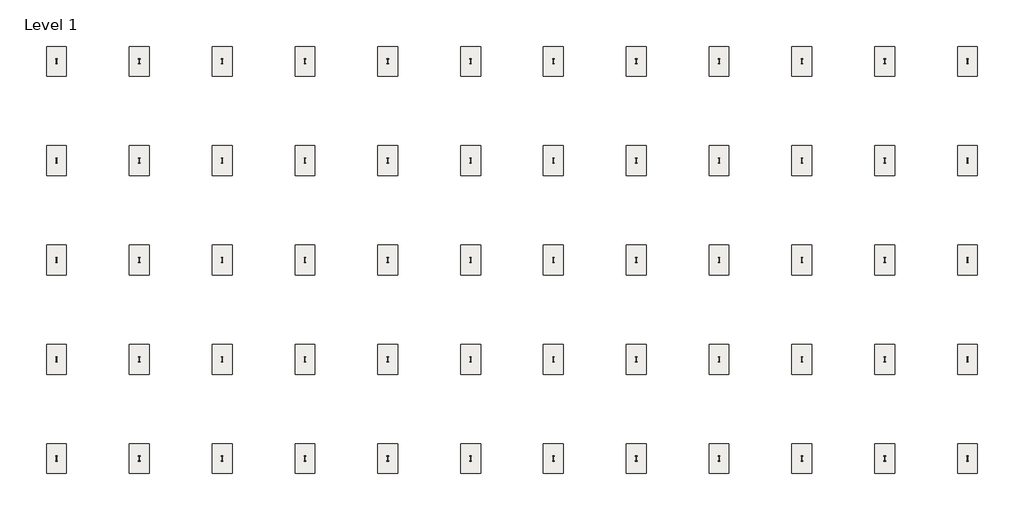
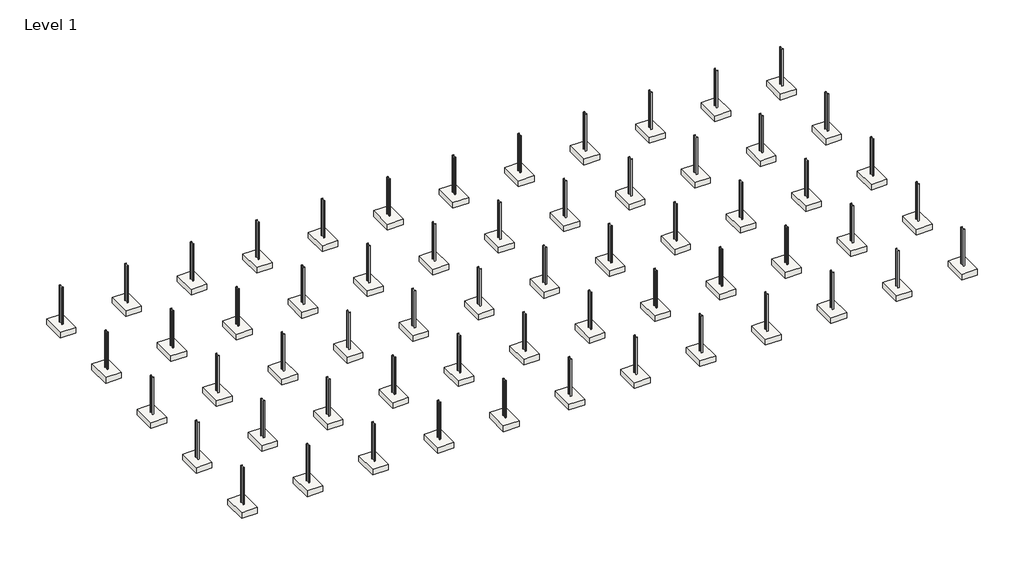
# One storey: 60 columns, 60 slabs.
"""IFC4 building model written with IfcOpenShell, lengths in millimetres."""

import ifcopenshell
import ifcopenshell.guid

model = None  # the IFC model being written
_history = None  # IfcOwnerHistory: only IFC2X3 demands one
_inside = {}  # id of a spatial element -> (the spatial element, [elements in it])
_under = {}  # id of a project, library or spatial element -> (it, [spatial elements below it])
_declared = {}  # id of a project -> (the project, [libraries it declares])
_typed = {}  # id of a type object -> (the type object, [elements of that type])
_made_of = {}  # id of a material, layer set ... -> (it, [elements and type objects made of it])


def new_model(schema):
    """Start an empty IFC model of exactly this schema.

    Asked for "IFC4X3", IfcOpenShell would pick the latest addendum, in which some entities
    have other attributes; the version numbers below select the first issue.
    IFC2X3 requires an IfcOwnerHistory on every rooted entity: one is made here for all.
    """
    global model, _history
    if schema == "IFC4X3":
        model = ifcopenshell.file(schema_version=(4, 3, 0, 0))
    else:
        model = ifcopenshell.file(schema=schema)
    _inside.clear()
    _under.clear()
    _declared.clear()
    _typed.clear()
    _made_of.clear()
    _history = None
    if model.schema == "IFC2X3":
        org = make("IfcOrganization", Name="unknown")
        user = make(
            "IfcPersonAndOrganization",
            ThePerson=make("IfcPerson", FamilyName="unknown"),
            TheOrganization=org,
        )
        app = make(
            "IfcApplication",
            ApplicationDeveloper=org,
            Version="unknown",
            ApplicationFullName="unknown",
            ApplicationIdentifier="unknown",
        )
        _history = make(
            "IfcOwnerHistory",
            OwningUser=user,
            OwningApplication=app,
            ChangeAction="ADDED",
            CreationDate=0,
        )
    return model


def make(cls, **values):
    """One entity of the class cls with the attributes given. An attribute that is None is left unset."""
    return model.create_entity(
        cls, **{name: value for name, value in values.items() if value is not None}
    )


def rooted(cls, **values):
    """An entity with a GlobalId (a new one), such as an element, a storey or a relation."""
    return make(cls, GlobalId=ifcopenshell.guid.new(), OwnerHistory=_history, **values)


def si_unit(unit_type, name, prefix=None):
    """IfcSIUnit, for example si_unit("LENGTHUNIT", "METRE", prefix="MILLI")."""
    return make("IfcSIUnit", UnitType=unit_type, Prefix=prefix, Name=name)


def assignment(units):
    """IfcUnitAssignment: the units of a project."""
    return None if units is None else make("IfcUnitAssignment", Units=units)


def point(xyz):
    """IfcCartesianPoint."""
    return None if xyz is None else make("IfcCartesianPoint", Coordinates=xyz)


def direction(xyz):
    """IfcDirection."""
    return None if xyz is None else make("IfcDirection", DirectionRatios=xyz)


def frame(location, z_axis=None, x_axis=None):
    """IfcAxis2Placement3D, a coordinate frame: its origin and axes. An axis left out is left unset."""
    return make(
        "IfcAxis2Placement3D",
        Location=point(location),
        Axis=direction(z_axis),
        RefDirection=direction(x_axis),
    )


def frame_2d(location, x_axis=None):
    """IfcAxis2Placement2D, a coordinate frame in the plane: its origin and x axis."""
    return make(
        "IfcAxis2Placement2D", Location=point(location), RefDirection=direction(x_axis)
    )


def origin():
    """The frame at (0, 0, 0) with its axes left unset."""
    return frame((0.0, 0.0, 0.0))


def origin_with_axes():
    """The frame at (0, 0, 0) with the z axis (0, 0, 1) and the x axis (1, 0, 0) written out."""
    return frame((0.0, 0.0, 0.0), z_axis=(0.0, 0.0, 1.0), x_axis=(1.0, 0.0, 0.0))


def place(relative_to, where):
    """IfcLocalPlacement: puts the frame where relative to a parent placement (None: the world)."""
    return make(
        "IfcLocalPlacement", PlacementRelTo=relative_to, RelativePlacement=where
    )


def context(
    kind, dimensions, precision=None, world=None, true_north=None, identifier=None
):
    """IfcGeometricRepresentationContext, for example the 3D "Model" context."""
    return make(
        "IfcGeometricRepresentationContext",
        ContextIdentifier=identifier,
        ContextType=kind,
        CoordinateSpaceDimension=dimensions,
        Precision=precision,
        WorldCoordinateSystem=world,
        TrueNorth=true_north,
    )


def project(units=None, contexts=None):
    """IfcProject with its units and contexts."""
    return rooted(
        "IfcProject",
        Name="project",
        RepresentationContexts=contexts,
        UnitsInContext=assignment(units),
    )


def spatial(cls, under=None, at=None, **own):
    """A site, building, storey or space (cls), placed at a placement, below another one or the project."""
    s = rooted(cls, ObjectPlacement=at, **own)
    if under is not None:
        _under.setdefault(under.id(), (under, []))[1].append(s)
    return s


def polyline(points):
    """IfcPolyline through the points."""
    return make("IfcPolyline", Points=[point(p) for p in points])


def circle_curve(where, radius):
    """IfcCircle in the frame where."""
    return make("IfcCircle", Position=where, Radius=radius)


def trimmed(basis, trim1, trim2, sense, master):
    """IfcTrimmedCurve: the piece of a basis curve between two trims."""
    return make(
        "IfcTrimmedCurve",
        BasisCurve=basis,
        Trim1=trim1,
        Trim2=trim2,
        SenseAgreement=sense,
        MasterRepresentation=master,
    )


def segment(curve, same_sense, transition):
    """IfcCompositeCurveSegment."""
    return make(
        "IfcCompositeCurveSegment",
        Transition=transition,
        SameSense=same_sense,
        ParentCurve=curve,
    )


def composite_curve(segments, self_intersect=None):
    """IfcCompositeCurve: segments joined end to end."""
    return make("IfcCompositeCurve", Segments=segments, SelfIntersect=self_intersect)


def outline(outer, holes=None, kind="AREA"):
    """IfcArbitraryClosedProfileDef: a profile drawn as a closed curve; with holes, ...WithVoids."""
    if holes is None:
        return make("IfcArbitraryClosedProfileDef", ProfileType=kind, OuterCurve=outer)
    return make(
        "IfcArbitraryProfileDefWithVoids",
        ProfileType=kind,
        OuterCurve=outer,
        InnerCurves=holes,
    )


def extrude(swept, where, along, depth):
    """IfcExtrudedAreaSolid: the profile swept, set in the frame where, extruded along a direction by depth."""
    return make(
        "IfcExtrudedAreaSolid",
        SweptArea=swept,
        Position=where,
        ExtrudedDirection=direction(along),
        Depth=depth,
    )


def shape(context_of_items, identifier, shape_type, items):
    """IfcShapeRepresentation: the items that make up one representation, for example the "Body"."""
    return make(
        "IfcShapeRepresentation",
        ContextOfItems=context_of_items,
        RepresentationIdentifier=identifier,
        RepresentationType=shape_type,
        Items=items,
    )


def source(mapping_origin, context_of_items, identifier, shape_type, items):
    """IfcRepresentationMap: a shape defined once, which mapped items show again and again."""
    return make(
        "IfcRepresentationMap",
        MappingOrigin=mapping_origin,
        MappedRepresentation=shape(context_of_items, identifier, shape_type, items),
    )


def transform(
    local_origin,
    x_axis=None,
    y_axis=None,
    z_axis=None,
    scale=None,
    scale2=None,
    scale3=None,
    uniform=True,
):
    """IfcCartesianTransformationOperator3D, or its non-uniform kind. x_axis, y_axis, z_axis: its Axis1, 2, 3."""
    if uniform:
        return make(
            "IfcCartesianTransformationOperator3D",
            Axis1=direction(x_axis),
            Axis2=direction(y_axis),
            LocalOrigin=point(local_origin),
            Scale=scale,
            Axis3=direction(z_axis),
        )
    return make(
        "IfcCartesianTransformationOperator3DnonUniform",
        Axis1=direction(x_axis),
        Axis2=direction(y_axis),
        LocalOrigin=point(local_origin),
        Scale=scale,
        Axis3=direction(z_axis),
        Scale2=scale2,
        Scale3=scale3,
    )


def mapped(mapping_source, mapping_target):
    """IfcMappedItem: shows the shape of a source again, moved by a transform."""
    return make(
        "IfcMappedItem", MappingSource=mapping_source, MappingTarget=mapping_target
    )


def made_of(thing, what):
    """Note that an element or type object is made of a material, layer set ...; save() writes the relation."""
    if what is not None:
        _made_of.setdefault(what.id(), (what, []))[1].append(thing)
    return thing


def element(
    cls,
    number,
    at=None,
    inside=None,
    cuts=None,
    type_object=None,
    material=None,
    context=None,
    identifier="Body",
    shape_type=None,
    held_by="IfcProductDefinitionShape",
    body=None,
    shapes=None,
    **own,
):
    """One element of the class cls, such as IfcWall. Its Tag is "e" and its number.

    at: its placement. inside: the storey or other place that contains it. cuts: it is an
    opening in that element (IfcRelVoidsElement). A single representation is given by context,
    identifier, shape_type and body (its items); several are given by shapes. held_by: the class
    of the entity that holds the representations. save() writes the other relations.
    """
    e = rooted(cls, Tag="e%d" % number, ObjectPlacement=at, **own)
    if body is not None:
        shapes = [shape(context, identifier, shape_type, body)]
    if shapes is not None:
        e.Representation = make(held_by, Representations=shapes)
    if inside is not None:
        _inside.setdefault(inside.id(), (inside, []))[1].append(e)
    if cuts is not None:
        rooted(
            "IfcRelVoidsElement", RelatingBuildingElement=cuts, RelatedOpeningElement=e
        )
    if type_object is not None:
        _typed.setdefault(type_object.id(), (type_object, []))[1].append(e)
    return made_of(e, material)


def aggregate(whole, parts):
    """IfcRelAggregates: a whole, such as a stair, and the parts it consists of."""
    return rooted("IfcRelAggregates", RelatingObject=whole, RelatedObjects=parts)


def save(model, path):
    """Write the relations noted so far, then the file.

    IfcRelAggregates (storeys below a building ...), IfcRelContainedInSpatialStructure (elements
    in a storey), IfcRelDefinesByType, IfcRelAssociatesMaterial and IfcRelDeclares: one each for
    every whole, place, type object, material and project.
    """
    for whole, parts in _under.values():
        aggregate(whole, parts)
    for where, things in _inside.values():
        rooted(
            "IfcRelContainedInSpatialStructure",
            RelatedElements=things,
            RelatingStructure=where,
        )
    for kind, things in _typed.values():
        rooted("IfcRelDefinesByType", RelatedObjects=things, RelatingType=kind)
    for what, things in _made_of.values():
        rooted("IfcRelAssociatesMaterial", RelatedObjects=things, RelatingMaterial=what)
    for by, libraries in _declared.values():
        rooted("IfcRelDeclares", RelatingContext=by, RelatedDefinitions=libraries)
    model.write(path)


def ub_universal_beams_column_ub305x102x25_abf45cfe(model_context):
    return source(origin(), model_context, "Body", "SweptSolid", [
        extrude(outline(composite_curve([segment(polyline([(50.8, 152.55), (50.8, 145.55), (10.5, 145.55)]), True, "CONTINUOUS"), segment(trimmed(circle_curve(frame_2d((10.5, 137.95)), 7.6), [point((10.5, 145.55))], [point((2.9, 137.95))], True, "CARTESIAN"), True, "CONTINUOUS"), segment(polyline([(2.9, 137.95), (2.9, -137.95)]), True, "CONTINUOUS"), segment(trimmed(circle_curve(frame_2d((10.5, -137.95)), 7.6), [point((2.9, -137.95))], [point((10.5, -145.55))], True, "CARTESIAN"), True, "CONTINUOUS"), segment(polyline([(10.5, -145.55), (50.8, -145.55), (50.8, -152.55), (-50.8, -152.55), (-50.8, -145.55), (-10.5, -145.55)]), True, "CONTINUOUS"), segment(trimmed(circle_curve(frame_2d((-10.5, -137.95)), 7.6), [point((-10.5, -145.55))], [point((-2.9, -137.95))], True, "CARTESIAN"), True, "CONTINUOUS"), segment(polyline([(-2.9, -137.95), (-2.9, 137.95)]), True, "CONTINUOUS"), segment(trimmed(circle_curve(frame_2d((-10.5, 137.95)), 7.6), [point((-2.9, 137.95))], [point((-10.5, 145.55))], True, "CARTESIAN"), True, "CONTINUOUS"), segment(polyline([(-10.5, 145.55), (-50.8, 145.55), (-50.8, 152.55), (50.8, 152.55)]), True, "CONTINUOUS")], self_intersect=False)), origin_with_axes(), (0.0, 0.0, 1.0), 3000.0),
    ])


def footing_rectangular_1800_x_1200_x_450mm_16ba7ea5(model_context):
    return source(origin(), model_context, "Body", "SweptSolid", [
        extrude(outline(polyline([(600.0, 900.0), (600.0, -900.0), (-600.0, -900.0), (-600.0, 900.0), (600.0, 900.0)])), frame((0.0, 0.0, -450.0), z_axis=(0.0, 0.0, 1.0), x_axis=(1.0, 0.0, 0.0)), (0.0, 0.0, 1.0), 450.0),
    ])


model = new_model("IFC4")

# Units and contexts
model_context = context("Model", 3, world=origin())
ifc_project = project(units=[si_unit("LENGTHUNIT", "METRE", prefix="MILLI")], contexts=[model_context])

# Site, building, storey
site = spatial("IfcSite", under=ifc_project)
building = spatial("IfcBuilding", under=site)
storey = spatial("IfcBuildingStorey", under=building, Name="Level 1", Elevation=0.0)

# Columns
placement = place(None, origin())
ub_universal_beams_column_ub305x102x25_shape = ub_universal_beams_column_ub305x102x25_abf45cfe(model_context)
element("IfcColumn", 1, ObjectType="UB-Universal Beams-Column : UB305x102x25", at=placement, inside=storey, context=model_context, shape_type="MappedRepresentation", body=[
    mapped(ub_universal_beams_column_ub305x102x25_shape, transform((0.0, 0.0, 0.0), x_axis=(-1.0, 0.0, 0.0), y_axis=(0.0, -1.0, 0.0), z_axis=(0.0, 0.0, 1.0))),
])
element("IfcColumn", 2, ObjectType="UB-Universal Beams-Column : UB305x102x25", at=placement, inside=storey, context=model_context, shape_type="MappedRepresentation", body=[
    mapped(ub_universal_beams_column_ub305x102x25_shape, transform((0.0, 6000.0, 0.0), x_axis=(-1.0, 0.0, 0.0), y_axis=(0.0, -1.0, 0.0), z_axis=(0.0, 0.0, 1.0))),
])
element("IfcColumn", 3, ObjectType="UB-Universal Beams-Column : UB305x102x25", at=placement, inside=storey, context=model_context, shape_type="MappedRepresentation", body=[
    mapped(ub_universal_beams_column_ub305x102x25_shape, transform((0.0, 12000.0, 0.0), x_axis=(-1.0, 0.0, 0.0), y_axis=(0.0, -1.0, 0.0), z_axis=(0.0, 0.0, 1.0))),
])
element("IfcColumn", 4, ObjectType="UB-Universal Beams-Column : UB305x102x25", at=placement, inside=storey, context=model_context, shape_type="MappedRepresentation", body=[
    mapped(ub_universal_beams_column_ub305x102x25_shape, transform((0.0, 18000.0, 0.0), x_axis=(-1.0, 0.0, 0.0), y_axis=(0.0, -1.0, 0.0), z_axis=(0.0, 0.0, 1.0))),
])
element("IfcColumn", 5, ObjectType="UB-Universal Beams-Column : UB305x102x25", at=placement, inside=storey, context=model_context, shape_type="MappedRepresentation", body=[
    mapped(ub_universal_beams_column_ub305x102x25_shape, transform((0.0, 24000.0, 0.0), x_axis=(-1.0, 0.0, 0.0), y_axis=(0.0, -1.0, 0.0), z_axis=(0.0, 0.0, 1.0))),
])
element("IfcColumn", 6, ObjectType="UB-Universal Beams-Column : UB305x102x25", at=placement, inside=storey, context=model_context, shape_type="MappedRepresentation", body=[
    mapped(ub_universal_beams_column_ub305x102x25_shape, transform((5000.0, 0.0, 0.0), x_axis=(-1.0, 0.0, 0.0), y_axis=(0.0, -1.0, 0.0), z_axis=(0.0, 0.0, 1.0))),
])
element("IfcColumn", 7, ObjectType="UB-Universal Beams-Column : UB305x102x25", at=placement, inside=storey, context=model_context, shape_type="MappedRepresentation", body=[
    mapped(ub_universal_beams_column_ub305x102x25_shape, transform((10000.0, 0.0, 0.0), x_axis=(-1.0, 0.0, 0.0), y_axis=(0.0, -1.0, 0.0), z_axis=(0.0, 0.0, 1.0))),
])
element("IfcColumn", 8, ObjectType="UB-Universal Beams-Column : UB305x102x25", at=placement, inside=storey, context=model_context, shape_type="MappedRepresentation", body=[
    mapped(ub_universal_beams_column_ub305x102x25_shape, transform((15000.0, 0.0, 0.0), x_axis=(-1.0, 0.0, 0.0), y_axis=(0.0, -1.0, 0.0), z_axis=(0.0, 0.0, 1.0))),
])
element("IfcColumn", 9, ObjectType="UB-Universal Beams-Column : UB305x102x25", at=placement, inside=storey, context=model_context, shape_type="MappedRepresentation", body=[
    mapped(ub_universal_beams_column_ub305x102x25_shape, transform((20000.0, 0.0, 0.0), x_axis=(-1.0, 0.0, 0.0), y_axis=(0.0, -1.0, 0.0), z_axis=(0.0, 0.0, 1.0))),
])
element("IfcColumn", 10, ObjectType="UB-Universal Beams-Column : UB305x102x25", at=placement, inside=storey, context=model_context, shape_type="MappedRepresentation", body=[
    mapped(ub_universal_beams_column_ub305x102x25_shape, transform((25000.0, 0.0, 0.0), x_axis=(-1.0, 0.0, 0.0), y_axis=(0.0, -1.0, 0.0), z_axis=(0.0, 0.0, 1.0))),
])
element("IfcColumn", 11, ObjectType="UB-Universal Beams-Column : UB305x102x25", at=placement, inside=storey, context=model_context, shape_type="MappedRepresentation", body=[
    mapped(ub_universal_beams_column_ub305x102x25_shape, transform((30000.0, 0.0, 0.0), x_axis=(-1.0, 0.0, 0.0), y_axis=(0.0, -1.0, 0.0), z_axis=(0.0, 0.0, 1.0))),
])
element("IfcColumn", 12, ObjectType="UB-Universal Beams-Column : UB305x102x25", at=placement, inside=storey, context=model_context, shape_type="MappedRepresentation", body=[
    mapped(ub_universal_beams_column_ub305x102x25_shape, transform((35000.0, 0.0, 0.0), x_axis=(-1.0, 0.0, 0.0), y_axis=(0.0, -1.0, 0.0), z_axis=(0.0, 0.0, 1.0))),
])
element("IfcColumn", 13, ObjectType="UB-Universal Beams-Column : UB305x102x25", at=placement, inside=storey, context=model_context, shape_type="MappedRepresentation", body=[
    mapped(ub_universal_beams_column_ub305x102x25_shape, transform((40000.0, 0.0, 0.0), x_axis=(-1.0, 0.0, 0.0), y_axis=(0.0, -1.0, 0.0), z_axis=(0.0, 0.0, 1.0))),
])
element("IfcColumn", 14, ObjectType="UB-Universal Beams-Column : UB305x102x25", at=placement, inside=storey, context=model_context, shape_type="MappedRepresentation", body=[
    mapped(ub_universal_beams_column_ub305x102x25_shape, transform((45000.0, 0.0, 0.0), x_axis=(-1.0, 0.0, 0.0), y_axis=(0.0, -1.0, 0.0), z_axis=(0.0, 0.0, 1.0))),
])
element("IfcColumn", 15, ObjectType="UB-Universal Beams-Column : UB305x102x25", at=placement, inside=storey, context=model_context, shape_type="MappedRepresentation", body=[
    mapped(ub_universal_beams_column_ub305x102x25_shape, transform((50000.0, 0.0, 0.0), x_axis=(-1.0, 0.0, 0.0), y_axis=(0.0, -1.0, 0.0), z_axis=(0.0, 0.0, 1.0))),
])
element("IfcColumn", 16, ObjectType="UB-Universal Beams-Column : UB305x102x25", at=placement, inside=storey, context=model_context, shape_type="MappedRepresentation", body=[
    mapped(ub_universal_beams_column_ub305x102x25_shape, transform((55000.0, 0.0, 0.0), x_axis=(-1.0, 0.0, 0.0), y_axis=(0.0, -1.0, 0.0), z_axis=(0.0, 0.0, 1.0))),
])
element("IfcColumn", 17, ObjectType="UB-Universal Beams-Column : UB305x102x25", at=placement, inside=storey, context=model_context, shape_type="MappedRepresentation", body=[
    mapped(ub_universal_beams_column_ub305x102x25_shape, transform((5000.0, 6000.0, 0.0), x_axis=(-1.0, 0.0, 0.0), y_axis=(0.0, -1.0, 0.0), z_axis=(0.0, 0.0, 1.0))),
])
element("IfcColumn", 18, ObjectType="UB-Universal Beams-Column : UB305x102x25", at=placement, inside=storey, context=model_context, shape_type="MappedRepresentation", body=[
    mapped(ub_universal_beams_column_ub305x102x25_shape, transform((5000.0, 12000.0, 0.0), x_axis=(-1.0, 0.0, 0.0), y_axis=(0.0, -1.0, 0.0), z_axis=(0.0, 0.0, 1.0))),
])
element("IfcColumn", 19, ObjectType="UB-Universal Beams-Column : UB305x102x25", at=placement, inside=storey, context=model_context, shape_type="MappedRepresentation", body=[
    mapped(ub_universal_beams_column_ub305x102x25_shape, transform((5000.0, 18000.0, 0.0), x_axis=(-1.0, 0.0, 0.0), y_axis=(0.0, -1.0, 0.0), z_axis=(0.0, 0.0, 1.0))),
])
element("IfcColumn", 20, ObjectType="UB-Universal Beams-Column : UB305x102x25", at=placement, inside=storey, context=model_context, shape_type="MappedRepresentation", body=[
    mapped(ub_universal_beams_column_ub305x102x25_shape, transform((5000.0, 24000.0, 0.0), x_axis=(-1.0, 0.0, 0.0), y_axis=(0.0, -1.0, 0.0), z_axis=(0.0, 0.0, 1.0))),
])
element("IfcColumn", 21, ObjectType="UB-Universal Beams-Column : UB305x102x25", at=placement, inside=storey, context=model_context, shape_type="MappedRepresentation", body=[
    mapped(ub_universal_beams_column_ub305x102x25_shape, transform((10000.0, 6000.0, 0.0), x_axis=(-1.0, 0.0, 0.0), y_axis=(0.0, -1.0, 0.0), z_axis=(0.0, 0.0, 1.0))),
])
element("IfcColumn", 22, ObjectType="UB-Universal Beams-Column : UB305x102x25", at=placement, inside=storey, context=model_context, shape_type="MappedRepresentation", body=[
    mapped(ub_universal_beams_column_ub305x102x25_shape, transform((10000.0, 12000.0, 0.0), x_axis=(-1.0, 0.0, 0.0), y_axis=(0.0, -1.0, 0.0), z_axis=(0.0, 0.0, 1.0))),
])
element("IfcColumn", 23, ObjectType="UB-Universal Beams-Column : UB305x102x25", at=placement, inside=storey, context=model_context, shape_type="MappedRepresentation", body=[
    mapped(ub_universal_beams_column_ub305x102x25_shape, transform((10000.0, 18000.0, 0.0), x_axis=(-1.0, 0.0, 0.0), y_axis=(0.0, -1.0, 0.0), z_axis=(0.0, 0.0, 1.0))),
])
element("IfcColumn", 24, ObjectType="UB-Universal Beams-Column : UB305x102x25", at=placement, inside=storey, context=model_context, shape_type="MappedRepresentation", body=[
    mapped(ub_universal_beams_column_ub305x102x25_shape, transform((10000.0, 24000.0, 0.0), x_axis=(-1.0, 0.0, 0.0), y_axis=(0.0, -1.0, 0.0), z_axis=(0.0, 0.0, 1.0))),
])
element("IfcColumn", 25, ObjectType="UB-Universal Beams-Column : UB305x102x25", at=placement, inside=storey, context=model_context, shape_type="MappedRepresentation", body=[
    mapped(ub_universal_beams_column_ub305x102x25_shape, transform((15000.0, 6000.0, 0.0), x_axis=(-1.0, 0.0, 0.0), y_axis=(0.0, -1.0, 0.0), z_axis=(0.0, 0.0, 1.0))),
])
element("IfcColumn", 26, ObjectType="UB-Universal Beams-Column : UB305x102x25", at=placement, inside=storey, context=model_context, shape_type="MappedRepresentation", body=[
    mapped(ub_universal_beams_column_ub305x102x25_shape, transform((15000.0, 12000.0, 0.0), x_axis=(-1.0, 0.0, 0.0), y_axis=(0.0, -1.0, 0.0), z_axis=(0.0, 0.0, 1.0))),
])
element("IfcColumn", 27, ObjectType="UB-Universal Beams-Column : UB305x102x25", at=placement, inside=storey, context=model_context, shape_type="MappedRepresentation", body=[
    mapped(ub_universal_beams_column_ub305x102x25_shape, transform((15000.0, 18000.0, 0.0), x_axis=(-1.0, 0.0, 0.0), y_axis=(0.0, -1.0, 0.0), z_axis=(0.0, 0.0, 1.0))),
])
element("IfcColumn", 28, ObjectType="UB-Universal Beams-Column : UB305x102x25", at=placement, inside=storey, context=model_context, shape_type="MappedRepresentation", body=[
    mapped(ub_universal_beams_column_ub305x102x25_shape, transform((15000.0, 24000.0, 0.0), x_axis=(-1.0, 0.0, 0.0), y_axis=(0.0, -1.0, 0.0), z_axis=(0.0, 0.0, 1.0))),
])
element("IfcColumn", 29, ObjectType="UB-Universal Beams-Column : UB305x102x25", at=placement, inside=storey, context=model_context, shape_type="MappedRepresentation", body=[
    mapped(ub_universal_beams_column_ub305x102x25_shape, transform((20000.0, 6000.0, 0.0), x_axis=(-1.0, 0.0, 0.0), y_axis=(0.0, -1.0, 0.0), z_axis=(0.0, 0.0, 1.0))),
])
element("IfcColumn", 30, ObjectType="UB-Universal Beams-Column : UB305x102x25", at=placement, inside=storey, context=model_context, shape_type="MappedRepresentation", body=[
    mapped(ub_universal_beams_column_ub305x102x25_shape, transform((20000.0, 12000.0, 0.0), x_axis=(-1.0, 0.0, 0.0), y_axis=(0.0, -1.0, 0.0), z_axis=(0.0, 0.0, 1.0))),
])
element("IfcColumn", 31, ObjectType="UB-Universal Beams-Column : UB305x102x25", at=placement, inside=storey, context=model_context, shape_type="MappedRepresentation", body=[
    mapped(ub_universal_beams_column_ub305x102x25_shape, transform((20000.0, 18000.0, 0.0), x_axis=(-1.0, 0.0, 0.0), y_axis=(0.0, -1.0, 0.0), z_axis=(0.0, 0.0, 1.0))),
])
element("IfcColumn", 32, ObjectType="UB-Universal Beams-Column : UB305x102x25", at=placement, inside=storey, context=model_context, shape_type="MappedRepresentation", body=[
    mapped(ub_universal_beams_column_ub305x102x25_shape, transform((20000.0, 24000.0, 0.0), x_axis=(-1.0, 0.0, 0.0), y_axis=(0.0, -1.0, 0.0), z_axis=(0.0, 0.0, 1.0))),
])
element("IfcColumn", 33, ObjectType="UB-Universal Beams-Column : UB305x102x25", at=placement, inside=storey, context=model_context, shape_type="MappedRepresentation", body=[
    mapped(ub_universal_beams_column_ub305x102x25_shape, transform((25000.0, 6000.0, 0.0), x_axis=(-1.0, 0.0, 0.0), y_axis=(0.0, -1.0, 0.0), z_axis=(0.0, 0.0, 1.0))),
])
element("IfcColumn", 34, ObjectType="UB-Universal Beams-Column : UB305x102x25", at=placement, inside=storey, context=model_context, shape_type="MappedRepresentation", body=[
    mapped(ub_universal_beams_column_ub305x102x25_shape, transform((25000.0, 12000.0, 0.0), x_axis=(-1.0, 0.0, 0.0), y_axis=(0.0, -1.0, 0.0), z_axis=(0.0, 0.0, 1.0))),
])
element("IfcColumn", 35, ObjectType="UB-Universal Beams-Column : UB305x102x25", at=placement, inside=storey, context=model_context, shape_type="MappedRepresentation", body=[
    mapped(ub_universal_beams_column_ub305x102x25_shape, transform((25000.0, 18000.0, 0.0), x_axis=(-1.0, 0.0, 0.0), y_axis=(0.0, -1.0, 0.0), z_axis=(0.0, 0.0, 1.0))),
])
element("IfcColumn", 36, ObjectType="UB-Universal Beams-Column : UB305x102x25", at=placement, inside=storey, context=model_context, shape_type="MappedRepresentation", body=[
    mapped(ub_universal_beams_column_ub305x102x25_shape, transform((25000.0, 24000.0, 0.0), x_axis=(-1.0, 0.0, 0.0), y_axis=(0.0, -1.0, 0.0), z_axis=(0.0, 0.0, 1.0))),
])
element("IfcColumn", 37, ObjectType="UB-Universal Beams-Column : UB305x102x25", at=placement, inside=storey, context=model_context, shape_type="MappedRepresentation", body=[
    mapped(ub_universal_beams_column_ub305x102x25_shape, transform((30000.0, 6000.0, 0.0), x_axis=(-1.0, 0.0, 0.0), y_axis=(0.0, -1.0, 0.0), z_axis=(0.0, 0.0, 1.0))),
])
element("IfcColumn", 38, ObjectType="UB-Universal Beams-Column : UB305x102x25", at=placement, inside=storey, context=model_context, shape_type="MappedRepresentation", body=[
    mapped(ub_universal_beams_column_ub305x102x25_shape, transform((30000.0, 12000.0, 0.0), x_axis=(-1.0, 0.0, 0.0), y_axis=(0.0, -1.0, 0.0), z_axis=(0.0, 0.0, 1.0))),
])
element("IfcColumn", 39, ObjectType="UB-Universal Beams-Column : UB305x102x25", at=placement, inside=storey, context=model_context, shape_type="MappedRepresentation", body=[
    mapped(ub_universal_beams_column_ub305x102x25_shape, transform((30000.0, 18000.0, 0.0), x_axis=(-1.0, 0.0, 0.0), y_axis=(0.0, -1.0, 0.0), z_axis=(0.0, 0.0, 1.0))),
])
element("IfcColumn", 40, ObjectType="UB-Universal Beams-Column : UB305x102x25", at=placement, inside=storey, context=model_context, shape_type="MappedRepresentation", body=[
    mapped(ub_universal_beams_column_ub305x102x25_shape, transform((30000.0, 24000.0, 0.0), x_axis=(-1.0, 0.0, 0.0), y_axis=(0.0, -1.0, 0.0), z_axis=(0.0, 0.0, 1.0))),
])
element("IfcColumn", 41, ObjectType="UB-Universal Beams-Column : UB305x102x25", at=placement, inside=storey, context=model_context, shape_type="MappedRepresentation", body=[
    mapped(ub_universal_beams_column_ub305x102x25_shape, transform((35000.0, 6000.0, 0.0), x_axis=(-1.0, 0.0, 0.0), y_axis=(0.0, -1.0, 0.0), z_axis=(0.0, 0.0, 1.0))),
])
element("IfcColumn", 42, ObjectType="UB-Universal Beams-Column : UB305x102x25", at=placement, inside=storey, context=model_context, shape_type="MappedRepresentation", body=[
    mapped(ub_universal_beams_column_ub305x102x25_shape, transform((35000.0, 12000.0, 0.0), x_axis=(-1.0, 0.0, 0.0), y_axis=(0.0, -1.0, 0.0), z_axis=(0.0, 0.0, 1.0))),
])
element("IfcColumn", 43, ObjectType="UB-Universal Beams-Column : UB305x102x25", at=placement, inside=storey, context=model_context, shape_type="MappedRepresentation", body=[
    mapped(ub_universal_beams_column_ub305x102x25_shape, transform((35000.0, 18000.0, 0.0), x_axis=(-1.0, 0.0, 0.0), y_axis=(0.0, -1.0, 0.0), z_axis=(0.0, 0.0, 1.0))),
])
element("IfcColumn", 44, ObjectType="UB-Universal Beams-Column : UB305x102x25", at=placement, inside=storey, context=model_context, shape_type="MappedRepresentation", body=[
    mapped(ub_universal_beams_column_ub305x102x25_shape, transform((35000.0, 24000.0, 0.0), x_axis=(-1.0, 0.0, 0.0), y_axis=(0.0, -1.0, 0.0), z_axis=(0.0, 0.0, 1.0))),
])
element("IfcColumn", 45, ObjectType="UB-Universal Beams-Column : UB305x102x25", at=placement, inside=storey, context=model_context, shape_type="MappedRepresentation", body=[
    mapped(ub_universal_beams_column_ub305x102x25_shape, transform((40000.0, 6000.0, 0.0), x_axis=(-1.0, 0.0, 0.0), y_axis=(0.0, -1.0, 0.0), z_axis=(0.0, 0.0, 1.0))),
])
element("IfcColumn", 46, ObjectType="UB-Universal Beams-Column : UB305x102x25", at=placement, inside=storey, context=model_context, shape_type="MappedRepresentation", body=[
    mapped(ub_universal_beams_column_ub305x102x25_shape, transform((40000.0, 12000.0, 0.0), x_axis=(-1.0, 0.0, 0.0), y_axis=(0.0, -1.0, 0.0), z_axis=(0.0, 0.0, 1.0))),
])
element("IfcColumn", 47, ObjectType="UB-Universal Beams-Column : UB305x102x25", at=placement, inside=storey, context=model_context, shape_type="MappedRepresentation", body=[
    mapped(ub_universal_beams_column_ub305x102x25_shape, transform((40000.0, 18000.0, 0.0), x_axis=(-1.0, 0.0, 0.0), y_axis=(0.0, -1.0, 0.0), z_axis=(0.0, 0.0, 1.0))),
])
element("IfcColumn", 48, ObjectType="UB-Universal Beams-Column : UB305x102x25", at=placement, inside=storey, context=model_context, shape_type="MappedRepresentation", body=[
    mapped(ub_universal_beams_column_ub305x102x25_shape, transform((40000.0, 24000.0, 0.0), x_axis=(-1.0, 0.0, 0.0), y_axis=(0.0, -1.0, 0.0), z_axis=(0.0, 0.0, 1.0))),
])
element("IfcColumn", 49, ObjectType="UB-Universal Beams-Column : UB305x102x25", at=placement, inside=storey, context=model_context, shape_type="MappedRepresentation", body=[
    mapped(ub_universal_beams_column_ub305x102x25_shape, transform((45000.0, 6000.0, 0.0), x_axis=(-1.0, 0.0, 0.0), y_axis=(0.0, -1.0, 0.0), z_axis=(0.0, 0.0, 1.0))),
])
element("IfcColumn", 50, ObjectType="UB-Universal Beams-Column : UB305x102x25", at=placement, inside=storey, context=model_context, shape_type="MappedRepresentation", body=[
    mapped(ub_universal_beams_column_ub305x102x25_shape, transform((45000.0, 12000.0, 0.0), x_axis=(-1.0, 0.0, 0.0), y_axis=(0.0, -1.0, 0.0), z_axis=(0.0, 0.0, 1.0))),
])
element("IfcColumn", 51, ObjectType="UB-Universal Beams-Column : UB305x102x25", at=placement, inside=storey, context=model_context, shape_type="MappedRepresentation", body=[
    mapped(ub_universal_beams_column_ub305x102x25_shape, transform((45000.0, 18000.0, 0.0), x_axis=(-1.0, 0.0, 0.0), y_axis=(0.0, -1.0, 0.0), z_axis=(0.0, 0.0, 1.0))),
])
element("IfcColumn", 52, ObjectType="UB-Universal Beams-Column : UB305x102x25", at=placement, inside=storey, context=model_context, shape_type="MappedRepresentation", body=[
    mapped(ub_universal_beams_column_ub305x102x25_shape, transform((45000.0, 24000.0, 0.0), x_axis=(-1.0, 0.0, 0.0), y_axis=(0.0, -1.0, 0.0), z_axis=(0.0, 0.0, 1.0))),
])
element("IfcColumn", 53, ObjectType="UB-Universal Beams-Column : UB305x102x25", at=placement, inside=storey, context=model_context, shape_type="MappedRepresentation", body=[
    mapped(ub_universal_beams_column_ub305x102x25_shape, transform((50000.0, 6000.0, 0.0), x_axis=(-1.0, 0.0, 0.0), y_axis=(0.0, -1.0, 0.0), z_axis=(0.0, 0.0, 1.0))),
])
element("IfcColumn", 54, ObjectType="UB-Universal Beams-Column : UB305x102x25", at=placement, inside=storey, context=model_context, shape_type="MappedRepresentation", body=[
    mapped(ub_universal_beams_column_ub305x102x25_shape, transform((50000.0, 12000.0, 0.0), x_axis=(-1.0, 0.0, 0.0), y_axis=(0.0, -1.0, 0.0), z_axis=(0.0, 0.0, 1.0))),
])
element("IfcColumn", 55, ObjectType="UB-Universal Beams-Column : UB305x102x25", at=placement, inside=storey, context=model_context, shape_type="MappedRepresentation", body=[
    mapped(ub_universal_beams_column_ub305x102x25_shape, transform((50000.0, 18000.0, 0.0), x_axis=(-1.0, 0.0, 0.0), y_axis=(0.0, -1.0, 0.0), z_axis=(0.0, 0.0, 1.0))),
])
element("IfcColumn", 56, ObjectType="UB-Universal Beams-Column : UB305x102x25", at=placement, inside=storey, context=model_context, shape_type="MappedRepresentation", body=[
    mapped(ub_universal_beams_column_ub305x102x25_shape, transform((50000.0, 24000.0, 0.0), x_axis=(-1.0, 0.0, 0.0), y_axis=(0.0, -1.0, 0.0), z_axis=(0.0, 0.0, 1.0))),
])
element("IfcColumn", 57, ObjectType="UB-Universal Beams-Column : UB305x102x25", at=placement, inside=storey, context=model_context, shape_type="MappedRepresentation", body=[
    mapped(ub_universal_beams_column_ub305x102x25_shape, transform((55000.0, 6000.0, 0.0), x_axis=(-1.0, 0.0, 0.0), y_axis=(0.0, -1.0, 0.0), z_axis=(0.0, 0.0, 1.0))),
])
element("IfcColumn", 58, ObjectType="UB-Universal Beams-Column : UB305x102x25", at=placement, inside=storey, context=model_context, shape_type="MappedRepresentation", body=[
    mapped(ub_universal_beams_column_ub305x102x25_shape, transform((55000.0, 12000.0, 0.0), x_axis=(-1.0, 0.0, 0.0), y_axis=(0.0, -1.0, 0.0), z_axis=(0.0, 0.0, 1.0))),
])
element("IfcColumn", 59, ObjectType="UB-Universal Beams-Column : UB305x102x25", at=placement, inside=storey, context=model_context, shape_type="MappedRepresentation", body=[
    mapped(ub_universal_beams_column_ub305x102x25_shape, transform((55000.0, 18000.0, 0.0), x_axis=(-1.0, 0.0, 0.0), y_axis=(0.0, -1.0, 0.0), z_axis=(0.0, 0.0, 1.0))),
])
element("IfcColumn", 60, ObjectType="UB-Universal Beams-Column : UB305x102x25", at=placement, inside=storey, context=model_context, shape_type="MappedRepresentation", body=[
    mapped(ub_universal_beams_column_ub305x102x25_shape, transform((55000.0, 24000.0, 0.0), x_axis=(-1.0, 0.0, 0.0), y_axis=(0.0, -1.0, 0.0), z_axis=(0.0, 0.0, 1.0))),
])

# Slabs
footing_rectangular_1800_x_1200_x_450mm_shape = footing_rectangular_1800_x_1200_x_450mm_16ba7ea5(model_context)
element("IfcSlab", 61, ObjectType="Footing-Rectangular : 1800 x 1200 x 450mm", at=placement, inside=storey, context=model_context, shape_type="MappedRepresentation", body=[
    mapped(footing_rectangular_1800_x_1200_x_450mm_shape, transform((0.0, 24000.0, 0.0), x_axis=(1.0, 0.0, 0.0), y_axis=(0.0, 1.0, 0.0), z_axis=(0.0, 0.0, 1.0))),
])
element("IfcSlab", 62, ObjectType="Footing-Rectangular : 1800 x 1200 x 450mm", at=placement, inside=storey, context=model_context, shape_type="MappedRepresentation", body=[
    mapped(footing_rectangular_1800_x_1200_x_450mm_shape, transform((5000.0, 24000.0, 0.0), x_axis=(1.0, 0.0, 0.0), y_axis=(0.0, 1.0, 0.0), z_axis=(0.0, 0.0, 1.0))),
])
element("IfcSlab", 63, ObjectType="Footing-Rectangular : 1800 x 1200 x 450mm", at=placement, inside=storey, context=model_context, shape_type="MappedRepresentation", body=[
    mapped(footing_rectangular_1800_x_1200_x_450mm_shape, transform((10000.0, 6000.0, 0.0), x_axis=(-1.0, 0.0, 0.0), y_axis=(0.0, -1.0, 0.0), z_axis=(0.0, 0.0, 1.0))),
])
element("IfcSlab", 64, ObjectType="Footing-Rectangular : 1800 x 1200 x 450mm", at=placement, inside=storey, context=model_context, shape_type="MappedRepresentation", body=[
    mapped(footing_rectangular_1800_x_1200_x_450mm_shape, transform((10000.0, 12000.0, 0.0), x_axis=(-1.0, 0.0, 0.0), y_axis=(0.0, -1.0, 0.0), z_axis=(0.0, 0.0, 1.0))),
])
element("IfcSlab", 65, ObjectType="Footing-Rectangular : 1800 x 1200 x 450mm", at=placement, inside=storey, context=model_context, shape_type="MappedRepresentation", body=[
    mapped(footing_rectangular_1800_x_1200_x_450mm_shape, transform((10000.0, 18000.0, 0.0), x_axis=(-1.0, 0.0, 0.0), y_axis=(0.0, -1.0, 0.0), z_axis=(0.0, 0.0, 1.0))),
])
element("IfcSlab", 66, ObjectType="Footing-Rectangular : 1800 x 1200 x 450mm", at=placement, inside=storey, context=model_context, shape_type="MappedRepresentation", body=[
    mapped(footing_rectangular_1800_x_1200_x_450mm_shape, transform((10000.0, 24000.0, 0.0), x_axis=(-1.0, 0.0, 0.0), y_axis=(0.0, -1.0, 0.0), z_axis=(0.0, 0.0, 1.0))),
])
element("IfcSlab", 67, ObjectType="Footing-Rectangular : 1800 x 1200 x 450mm", at=placement, inside=storey, context=model_context, shape_type="MappedRepresentation", body=[
    mapped(footing_rectangular_1800_x_1200_x_450mm_shape, transform((15000.0, 6000.0, 0.0), x_axis=(-1.0, 0.0, 0.0), y_axis=(0.0, -1.0, 0.0), z_axis=(0.0, 0.0, 1.0))),
])
element("IfcSlab", 68, ObjectType="Footing-Rectangular : 1800 x 1200 x 450mm", at=placement, inside=storey, context=model_context, shape_type="MappedRepresentation", body=[
    mapped(footing_rectangular_1800_x_1200_x_450mm_shape, transform((15000.0, 12000.0, 0.0), x_axis=(-1.0, 0.0, 0.0), y_axis=(0.0, -1.0, 0.0), z_axis=(0.0, 0.0, 1.0))),
])
element("IfcSlab", 69, ObjectType="Footing-Rectangular : 1800 x 1200 x 450mm", at=placement, inside=storey, context=model_context, shape_type="MappedRepresentation", body=[
    mapped(footing_rectangular_1800_x_1200_x_450mm_shape, transform((15000.0, 18000.0, 0.0), x_axis=(-1.0, 0.0, 0.0), y_axis=(0.0, -1.0, 0.0), z_axis=(0.0, 0.0, 1.0))),
])
element("IfcSlab", 70, ObjectType="Footing-Rectangular : 1800 x 1200 x 450mm", at=placement, inside=storey, context=model_context, shape_type="MappedRepresentation", body=[
    mapped(footing_rectangular_1800_x_1200_x_450mm_shape, transform((15000.0, 24000.0, 0.0), x_axis=(-1.0, 0.0, 0.0), y_axis=(0.0, -1.0, 0.0), z_axis=(0.0, 0.0, 1.0))),
])
element("IfcSlab", 71, ObjectType="Footing-Rectangular : 1800 x 1200 x 450mm", at=placement, inside=storey, context=model_context, shape_type="MappedRepresentation", body=[
    mapped(footing_rectangular_1800_x_1200_x_450mm_shape, transform((20000.0, 6000.0, 0.0), x_axis=(-1.0, 0.0, 0.0), y_axis=(0.0, -1.0, 0.0), z_axis=(0.0, 0.0, 1.0))),
])
element("IfcSlab", 72, ObjectType="Footing-Rectangular : 1800 x 1200 x 450mm", at=placement, inside=storey, context=model_context, shape_type="MappedRepresentation", body=[
    mapped(footing_rectangular_1800_x_1200_x_450mm_shape, transform((20000.0, 12000.0, 0.0), x_axis=(-1.0, 0.0, 0.0), y_axis=(0.0, -1.0, 0.0), z_axis=(0.0, 0.0, 1.0))),
])
element("IfcSlab", 73, ObjectType="Footing-Rectangular : 1800 x 1200 x 450mm", at=placement, inside=storey, context=model_context, shape_type="MappedRepresentation", body=[
    mapped(footing_rectangular_1800_x_1200_x_450mm_shape, transform((20000.0, 18000.0, 0.0), x_axis=(-1.0, 0.0, 0.0), y_axis=(0.0, -1.0, 0.0), z_axis=(0.0, 0.0, 1.0))),
])
element("IfcSlab", 74, ObjectType="Footing-Rectangular : 1800 x 1200 x 450mm", at=placement, inside=storey, context=model_context, shape_type="MappedRepresentation", body=[
    mapped(footing_rectangular_1800_x_1200_x_450mm_shape, transform((20000.0, 24000.0, 0.0), x_axis=(-1.0, 0.0, 0.0), y_axis=(0.0, -1.0, 0.0), z_axis=(0.0, 0.0, 1.0))),
])
element("IfcSlab", 75, ObjectType="Footing-Rectangular : 1800 x 1200 x 450mm", at=placement, inside=storey, context=model_context, shape_type="MappedRepresentation", body=[
    mapped(footing_rectangular_1800_x_1200_x_450mm_shape, transform((25000.0, 6000.0, 0.0), x_axis=(-1.0, 0.0, 0.0), y_axis=(0.0, -1.0, 0.0), z_axis=(0.0, 0.0, 1.0))),
])
element("IfcSlab", 76, ObjectType="Footing-Rectangular : 1800 x 1200 x 450mm", at=placement, inside=storey, context=model_context, shape_type="MappedRepresentation", body=[
    mapped(footing_rectangular_1800_x_1200_x_450mm_shape, transform((25000.0, 12000.0, 0.0), x_axis=(-1.0, 0.0, 0.0), y_axis=(0.0, -1.0, 0.0), z_axis=(0.0, 0.0, 1.0))),
])
element("IfcSlab", 77, ObjectType="Footing-Rectangular : 1800 x 1200 x 450mm", at=placement, inside=storey, context=model_context, shape_type="MappedRepresentation", body=[
    mapped(footing_rectangular_1800_x_1200_x_450mm_shape, transform((25000.0, 18000.0, 0.0), x_axis=(-1.0, 0.0, 0.0), y_axis=(0.0, -1.0, 0.0), z_axis=(0.0, 0.0, 1.0))),
])
element("IfcSlab", 78, ObjectType="Footing-Rectangular : 1800 x 1200 x 450mm", at=placement, inside=storey, context=model_context, shape_type="MappedRepresentation", body=[
    mapped(footing_rectangular_1800_x_1200_x_450mm_shape, transform((25000.0, 24000.0, 0.0), x_axis=(-1.0, 0.0, 0.0), y_axis=(0.0, -1.0, 0.0), z_axis=(0.0, 0.0, 1.0))),
])
element("IfcSlab", 79, ObjectType="Footing-Rectangular : 1800 x 1200 x 450mm", at=placement, inside=storey, context=model_context, shape_type="MappedRepresentation", body=[
    mapped(footing_rectangular_1800_x_1200_x_450mm_shape, transform((30000.0, 6000.0, 0.0), x_axis=(-1.0, 0.0, 0.0), y_axis=(0.0, -1.0, 0.0), z_axis=(0.0, 0.0, 1.0))),
])
element("IfcSlab", 80, ObjectType="Footing-Rectangular : 1800 x 1200 x 450mm", at=placement, inside=storey, context=model_context, shape_type="MappedRepresentation", body=[
    mapped(footing_rectangular_1800_x_1200_x_450mm_shape, transform((30000.0, 12000.0, 0.0), x_axis=(-1.0, 0.0, 0.0), y_axis=(0.0, -1.0, 0.0), z_axis=(0.0, 0.0, 1.0))),
])
element("IfcSlab", 81, ObjectType="Footing-Rectangular : 1800 x 1200 x 450mm", at=placement, inside=storey, context=model_context, shape_type="MappedRepresentation", body=[
    mapped(footing_rectangular_1800_x_1200_x_450mm_shape, transform((30000.0, 18000.0, 0.0), x_axis=(-1.0, 0.0, 0.0), y_axis=(0.0, -1.0, 0.0), z_axis=(0.0, 0.0, 1.0))),
])
element("IfcSlab", 82, ObjectType="Footing-Rectangular : 1800 x 1200 x 450mm", at=placement, inside=storey, context=model_context, shape_type="MappedRepresentation", body=[
    mapped(footing_rectangular_1800_x_1200_x_450mm_shape, transform((30000.0, 24000.0, 0.0), x_axis=(-1.0, 0.0, 0.0), y_axis=(0.0, -1.0, 0.0), z_axis=(0.0, 0.0, 1.0))),
])
element("IfcSlab", 83, ObjectType="Footing-Rectangular : 1800 x 1200 x 450mm", at=placement, inside=storey, context=model_context, shape_type="MappedRepresentation", body=[
    mapped(footing_rectangular_1800_x_1200_x_450mm_shape, transform((35000.0, 6000.0, 0.0), x_axis=(-1.0, 0.0, 0.0), y_axis=(0.0, -1.0, 0.0), z_axis=(0.0, 0.0, 1.0))),
])
element("IfcSlab", 84, ObjectType="Footing-Rectangular : 1800 x 1200 x 450mm", at=placement, inside=storey, context=model_context, shape_type="MappedRepresentation", body=[
    mapped(footing_rectangular_1800_x_1200_x_450mm_shape, transform((35000.0, 12000.0, 0.0), x_axis=(-1.0, 0.0, 0.0), y_axis=(0.0, -1.0, 0.0), z_axis=(0.0, 0.0, 1.0))),
])
element("IfcSlab", 85, ObjectType="Footing-Rectangular : 1800 x 1200 x 450mm", at=placement, inside=storey, context=model_context, shape_type="MappedRepresentation", body=[
    mapped(footing_rectangular_1800_x_1200_x_450mm_shape, transform((35000.0, 18000.0, 0.0), x_axis=(-1.0, 0.0, 0.0), y_axis=(0.0, -1.0, 0.0), z_axis=(0.0, 0.0, 1.0))),
])
element("IfcSlab", 86, ObjectType="Footing-Rectangular : 1800 x 1200 x 450mm", at=placement, inside=storey, context=model_context, shape_type="MappedRepresentation", body=[
    mapped(footing_rectangular_1800_x_1200_x_450mm_shape, transform((35000.0, 24000.0, 0.0), x_axis=(-1.0, 0.0, 0.0), y_axis=(0.0, -1.0, 0.0), z_axis=(0.0, 0.0, 1.0))),
])
element("IfcSlab", 87, ObjectType="Footing-Rectangular : 1800 x 1200 x 450mm", at=placement, inside=storey, context=model_context, shape_type="MappedRepresentation", body=[
    mapped(footing_rectangular_1800_x_1200_x_450mm_shape, transform((40000.0, 6000.0, 0.0), x_axis=(-1.0, 0.0, 0.0), y_axis=(0.0, -1.0, 0.0), z_axis=(0.0, 0.0, 1.0))),
])
element("IfcSlab", 88, ObjectType="Footing-Rectangular : 1800 x 1200 x 450mm", at=placement, inside=storey, context=model_context, shape_type="MappedRepresentation", body=[
    mapped(footing_rectangular_1800_x_1200_x_450mm_shape, transform((40000.0, 12000.0, 0.0), x_axis=(-1.0, 0.0, 0.0), y_axis=(0.0, -1.0, 0.0), z_axis=(0.0, 0.0, 1.0))),
])
element("IfcSlab", 89, ObjectType="Footing-Rectangular : 1800 x 1200 x 450mm", at=placement, inside=storey, context=model_context, shape_type="MappedRepresentation", body=[
    mapped(footing_rectangular_1800_x_1200_x_450mm_shape, transform((40000.0, 18000.0, 0.0), x_axis=(-1.0, 0.0, 0.0), y_axis=(0.0, -1.0, 0.0), z_axis=(0.0, 0.0, 1.0))),
])
element("IfcSlab", 90, ObjectType="Footing-Rectangular : 1800 x 1200 x 450mm", at=placement, inside=storey, context=model_context, shape_type="MappedRepresentation", body=[
    mapped(footing_rectangular_1800_x_1200_x_450mm_shape, transform((40000.0, 24000.0, 0.0), x_axis=(-1.0, 0.0, 0.0), y_axis=(0.0, -1.0, 0.0), z_axis=(0.0, 0.0, 1.0))),
])
element("IfcSlab", 91, ObjectType="Footing-Rectangular : 1800 x 1200 x 450mm", at=placement, inside=storey, context=model_context, shape_type="MappedRepresentation", body=[
    mapped(footing_rectangular_1800_x_1200_x_450mm_shape, transform((45000.0, 6000.0, 0.0), x_axis=(-1.0, 0.0, 0.0), y_axis=(0.0, -1.0, 0.0), z_axis=(0.0, 0.0, 1.0))),
])
element("IfcSlab", 92, ObjectType="Footing-Rectangular : 1800 x 1200 x 450mm", at=placement, inside=storey, context=model_context, shape_type="MappedRepresentation", body=[
    mapped(footing_rectangular_1800_x_1200_x_450mm_shape, transform((45000.0, 12000.0, 0.0), x_axis=(-1.0, 0.0, 0.0), y_axis=(0.0, -1.0, 0.0), z_axis=(0.0, 0.0, 1.0))),
])
element("IfcSlab", 93, ObjectType="Footing-Rectangular : 1800 x 1200 x 450mm", at=placement, inside=storey, context=model_context, shape_type="MappedRepresentation", body=[
    mapped(footing_rectangular_1800_x_1200_x_450mm_shape, transform((45000.0, 18000.0, 0.0), x_axis=(-1.0, 0.0, 0.0), y_axis=(0.0, -1.0, 0.0), z_axis=(0.0, 0.0, 1.0))),
])
element("IfcSlab", 94, ObjectType="Footing-Rectangular : 1800 x 1200 x 450mm", at=placement, inside=storey, context=model_context, shape_type="MappedRepresentation", body=[
    mapped(footing_rectangular_1800_x_1200_x_450mm_shape, transform((45000.0, 24000.0, 0.0), x_axis=(-1.0, 0.0, 0.0), y_axis=(0.0, -1.0, 0.0), z_axis=(0.0, 0.0, 1.0))),
])
element("IfcSlab", 95, ObjectType="Footing-Rectangular : 1800 x 1200 x 450mm", at=placement, inside=storey, context=model_context, shape_type="MappedRepresentation", body=[
    mapped(footing_rectangular_1800_x_1200_x_450mm_shape, transform((50000.0, 6000.0, 0.0), x_axis=(-1.0, 0.0, 0.0), y_axis=(0.0, -1.0, 0.0), z_axis=(0.0, 0.0, 1.0))),
])
element("IfcSlab", 96, ObjectType="Footing-Rectangular : 1800 x 1200 x 450mm", at=placement, inside=storey, context=model_context, shape_type="MappedRepresentation", body=[
    mapped(footing_rectangular_1800_x_1200_x_450mm_shape, transform((50000.0, 12000.0, 0.0), x_axis=(-1.0, 0.0, 0.0), y_axis=(0.0, -1.0, 0.0), z_axis=(0.0, 0.0, 1.0))),
])
element("IfcSlab", 97, ObjectType="Footing-Rectangular : 1800 x 1200 x 450mm", at=placement, inside=storey, context=model_context, shape_type="MappedRepresentation", body=[
    mapped(footing_rectangular_1800_x_1200_x_450mm_shape, transform((50000.0, 18000.0, 0.0), x_axis=(-1.0, 0.0, 0.0), y_axis=(0.0, -1.0, 0.0), z_axis=(0.0, 0.0, 1.0))),
])
element("IfcSlab", 98, ObjectType="Footing-Rectangular : 1800 x 1200 x 450mm", at=placement, inside=storey, context=model_context, shape_type="MappedRepresentation", body=[
    mapped(footing_rectangular_1800_x_1200_x_450mm_shape, transform((50000.0, 24000.0, 0.0), x_axis=(-1.0, 0.0, 0.0), y_axis=(0.0, -1.0, 0.0), z_axis=(0.0, 0.0, 1.0))),
])
element("IfcSlab", 99, ObjectType="Footing-Rectangular : 1800 x 1200 x 450mm", at=placement, inside=storey, context=model_context, shape_type="MappedRepresentation", body=[
    mapped(footing_rectangular_1800_x_1200_x_450mm_shape, transform((55000.0, 6000.0, 0.0), x_axis=(-1.0, 0.0, 0.0), y_axis=(0.0, -1.0, 0.0), z_axis=(0.0, 0.0, 1.0))),
])
element("IfcSlab", 100, ObjectType="Footing-Rectangular : 1800 x 1200 x 450mm", at=placement, inside=storey, context=model_context, shape_type="MappedRepresentation", body=[
    mapped(footing_rectangular_1800_x_1200_x_450mm_shape, transform((55000.0, 12000.0, 0.0), x_axis=(-1.0, 0.0, 0.0), y_axis=(0.0, -1.0, 0.0), z_axis=(0.0, 0.0, 1.0))),
])
element("IfcSlab", 101, ObjectType="Footing-Rectangular : 1800 x 1200 x 450mm", at=placement, inside=storey, context=model_context, shape_type="MappedRepresentation", body=[
    mapped(footing_rectangular_1800_x_1200_x_450mm_shape, transform((55000.0, 18000.0, 0.0), x_axis=(-1.0, 0.0, 0.0), y_axis=(0.0, -1.0, 0.0), z_axis=(0.0, 0.0, 1.0))),
])
element("IfcSlab", 102, ObjectType="Footing-Rectangular : 1800 x 1200 x 450mm", at=placement, inside=storey, context=model_context, shape_type="MappedRepresentation", body=[
    mapped(footing_rectangular_1800_x_1200_x_450mm_shape, transform((55000.0, 24000.0, 0.0), x_axis=(-1.0, 0.0, 0.0), y_axis=(0.0, -1.0, 0.0), z_axis=(0.0, 0.0, 1.0))),
])
element("IfcSlab", 103, ObjectType="Footing-Rectangular : 1800 x 1200 x 450mm", at=placement, inside=storey, context=model_context, shape_type="MappedRepresentation", body=[
    mapped(footing_rectangular_1800_x_1200_x_450mm_shape, transform((0.0, 18000.0, 0.0), x_axis=(1.0, 0.0, 0.0), y_axis=(0.0, 1.0, 0.0), z_axis=(0.0, 0.0, 1.0))),
])
element("IfcSlab", 104, ObjectType="Footing-Rectangular : 1800 x 1200 x 450mm", at=placement, inside=storey, context=model_context, shape_type="MappedRepresentation", body=[
    mapped(footing_rectangular_1800_x_1200_x_450mm_shape, transform((5000.0, 18000.0, 0.0), x_axis=(1.0, 0.0, 0.0), y_axis=(0.0, 1.0, 0.0), z_axis=(0.0, 0.0, 1.0))),
])
element("IfcSlab", 105, ObjectType="Footing-Rectangular : 1800 x 1200 x 450mm", at=placement, inside=storey, context=model_context, shape_type="MappedRepresentation", body=[
    mapped(footing_rectangular_1800_x_1200_x_450mm_shape, transform((5000.0, 12000.0, 0.0), x_axis=(1.0, 0.0, 0.0), y_axis=(0.0, 1.0, 0.0), z_axis=(0.0, 0.0, 1.0))),
])
element("IfcSlab", 106, ObjectType="Footing-Rectangular : 1800 x 1200 x 450mm", at=placement, inside=storey, context=model_context, shape_type="MappedRepresentation", body=[
    mapped(footing_rectangular_1800_x_1200_x_450mm_shape, transform((0.0, 12000.0, 0.0), x_axis=(1.0, 0.0, 0.0), y_axis=(0.0, 1.0, 0.0), z_axis=(0.0, 0.0, 1.0))),
])
element("IfcSlab", 107, ObjectType="Footing-Rectangular : 1800 x 1200 x 450mm", at=placement, inside=storey, context=model_context, shape_type="MappedRepresentation", body=[
    mapped(footing_rectangular_1800_x_1200_x_450mm_shape, transform((0.0, 6000.0, 0.0), x_axis=(1.0, 0.0, 0.0), y_axis=(0.0, 1.0, 0.0), z_axis=(0.0, 0.0, 1.0))),
])
element("IfcSlab", 108, ObjectType="Footing-Rectangular : 1800 x 1200 x 450mm", at=placement, inside=storey, context=model_context, shape_type="MappedRepresentation", body=[
    mapped(footing_rectangular_1800_x_1200_x_450mm_shape, transform((5000.0, 6000.0, 0.0), x_axis=(1.0, 0.0, 0.0), y_axis=(0.0, 1.0, 0.0), z_axis=(0.0, 0.0, 1.0))),
])
element("IfcSlab", 109, ObjectType="Footing-Rectangular : 1800 x 1200 x 450mm", at=placement, inside=storey, context=model_context, shape_type="MappedRepresentation", body=[
    mapped(footing_rectangular_1800_x_1200_x_450mm_shape, transform((5000.0, 0.0, 0.0), x_axis=(1.0, 0.0, 0.0), y_axis=(0.0, 1.0, 0.0), z_axis=(0.0, 0.0, 1.0))),
])
element("IfcSlab", 110, ObjectType="Footing-Rectangular : 1800 x 1200 x 450mm", at=placement, inside=storey, context=model_context, shape_type="MappedRepresentation", body=[
    mapped(footing_rectangular_1800_x_1200_x_450mm_shape, transform((10000.0, 0.0, 0.0), x_axis=(1.0, 0.0, 0.0), y_axis=(0.0, 1.0, 0.0), z_axis=(0.0, 0.0, 1.0))),
])
element("IfcSlab", 111, ObjectType="Footing-Rectangular : 1800 x 1200 x 450mm", at=placement, inside=storey, context=model_context, shape_type="MappedRepresentation", body=[
    mapped(footing_rectangular_1800_x_1200_x_450mm_shape, transform((15000.0, 0.0, 0.0), x_axis=(1.0, 0.0, 0.0), y_axis=(0.0, 1.0, 0.0), z_axis=(0.0, 0.0, 1.0))),
])
element("IfcSlab", 112, ObjectType="Footing-Rectangular : 1800 x 1200 x 450mm", at=placement, inside=storey, context=model_context, shape_type="MappedRepresentation", body=[
    mapped(footing_rectangular_1800_x_1200_x_450mm_shape, transform((0.0, 0.0, 0.0), x_axis=(1.0, 0.0, 0.0), y_axis=(0.0, 1.0, 0.0), z_axis=(0.0, 0.0, 1.0))),
])
element("IfcSlab", 113, ObjectType="Footing-Rectangular : 1800 x 1200 x 450mm", at=placement, inside=storey, context=model_context, shape_type="MappedRepresentation", body=[
    mapped(footing_rectangular_1800_x_1200_x_450mm_shape, transform((20000.0, 0.0, 0.0), x_axis=(1.0, 0.0, 0.0), y_axis=(0.0, 1.0, 0.0), z_axis=(0.0, 0.0, 1.0))),
])
element("IfcSlab", 114, ObjectType="Footing-Rectangular : 1800 x 1200 x 450mm", at=placement, inside=storey, context=model_context, shape_type="MappedRepresentation", body=[
    mapped(footing_rectangular_1800_x_1200_x_450mm_shape, transform((25000.0, 0.0, 0.0), x_axis=(1.0, 0.0, 0.0), y_axis=(0.0, 1.0, 0.0), z_axis=(0.0, 0.0, 1.0))),
])
element("IfcSlab", 115, ObjectType="Footing-Rectangular : 1800 x 1200 x 450mm", at=placement, inside=storey, context=model_context, shape_type="MappedRepresentation", body=[
    mapped(footing_rectangular_1800_x_1200_x_450mm_shape, transform((30000.0, 0.0, 0.0), x_axis=(1.0, 0.0, 0.0), y_axis=(0.0, 1.0, 0.0), z_axis=(0.0, 0.0, 1.0))),
])
element("IfcSlab", 116, ObjectType="Footing-Rectangular : 1800 x 1200 x 450mm", at=placement, inside=storey, context=model_context, shape_type="MappedRepresentation", body=[
    mapped(footing_rectangular_1800_x_1200_x_450mm_shape, transform((35000.0, 0.0, 0.0), x_axis=(1.0, 0.0, 0.0), y_axis=(0.0, 1.0, 0.0), z_axis=(0.0, 0.0, 1.0))),
])
element("IfcSlab", 117, ObjectType="Footing-Rectangular : 1800 x 1200 x 450mm", at=placement, inside=storey, context=model_context, shape_type="MappedRepresentation", body=[
    mapped(footing_rectangular_1800_x_1200_x_450mm_shape, transform((40000.0, 0.0, 0.0), x_axis=(1.0, 0.0, 0.0), y_axis=(0.0, 1.0, 0.0), z_axis=(0.0, 0.0, 1.0))),
])
element("IfcSlab", 118, ObjectType="Footing-Rectangular : 1800 x 1200 x 450mm", at=placement, inside=storey, context=model_context, shape_type="MappedRepresentation", body=[
    mapped(footing_rectangular_1800_x_1200_x_450mm_shape, transform((45000.0, 0.0, 0.0), x_axis=(1.0, 0.0, 0.0), y_axis=(0.0, 1.0, 0.0), z_axis=(0.0, 0.0, 1.0))),
])
element("IfcSlab", 119, ObjectType="Footing-Rectangular : 1800 x 1200 x 450mm", at=placement, inside=storey, context=model_context, shape_type="MappedRepresentation", body=[
    mapped(footing_rectangular_1800_x_1200_x_450mm_shape, transform((50000.0, 0.0, 0.0), x_axis=(1.0, 0.0, 0.0), y_axis=(0.0, 1.0, 0.0), z_axis=(0.0, 0.0, 1.0))),
])
element("IfcSlab", 120, ObjectType="Footing-Rectangular : 1800 x 1200 x 450mm", at=placement, inside=storey, context=model_context, shape_type="MappedRepresentation", body=[
    mapped(footing_rectangular_1800_x_1200_x_450mm_shape, transform((55000.0, 0.0, 0.0), x_axis=(1.0, 0.0, 0.0), y_axis=(0.0, 1.0, 0.0), z_axis=(0.0, 0.0, 1.0))),
])

save(model, "model.ifc")

# Revit data of these elements
# Project information
#   Project Issue Date = "Issue Date"
#   Project Status = "Project Status"
#   Client Name = "Owner"
#   Project Address = "Enter address here"
#   Project Name = "Project Name"
#   Project Number = "Project Number"
# Grids (mm)
#   "1": line (0, -6672.997) -> (0, 29554.368)
#   "A": line (-6601.463, 0) -> (61912.867, 0)
#   "2": line (5000, -6672.997) -> (5000, 29554.368)
#   "3": line (10000, -6672.997) -> (10000, 29554.368)
#   "4": line (15000, -6672.997) -> (15000, 29554.368)
#   "5": line (20000, -6672.997) -> (20000, 29554.368)
#   "6": line (25000, -6672.997) -> (25000, 29554.368)
#   "7": line (30000, -6672.997) -> (30000, 29554.368)
#   "8": line (35000, -6672.997) -> (35000, 29554.368)
#   "9": line (40000, -6672.997) -> (40000, 29554.368)
#   "10": line (45000, -6672.997) -> (45000, 29554.368)
#   "11": line (50000, -6672.997) -> (50000, 29554.368)
#   "12": line (55000, -6672.997) -> (55000, 29554.368)
#   "B": line (-6601.463, 6000) -> (61912.867, 6000)
#   "C": line (-6601.463, 12000) -> (61912.867, 12000)
#   "D": line (-6601.463, 18000) -> (61912.867, 18000)
#   "E": line (-6601.463, 24000) -> (61912.867, 24000)
# Type "UB-Universal Beams-Column : UB305x102x25"
#   Section Name Key = "UB305X102X25"
#   Width = 101.6 mm
#   Web Thickness = 5.8 mm
#   Web Fillet = 7.6 mm
#   Warping Constant = 27300 cm⁶
#   Torsional Moment of Inertia = 4.77 cm⁴
#   Section Area = 31.6 cm²
#   Plastic Modulus weak axis = 0.00137727 (stored number, unit not read)
#   Plastic Modulus strong axis = 0.0120776 (stored number, unit not read)
#   Nominal Weight = 243.204 N/m
#   Moment of Inertia weak axis = 123 cm⁴
#   Moment of Inertia strong axis = 4455 cm⁴
#   Height = 305.1 mm
#   Flange Thickness = 7 mm
#   Elastic Modulus weak axis = 0.000854615 (stored number, unit not read)
#   Elastic Modulus strong axis = 0.0103119 (stored number, unit not read)
#   Centroid Vertical = 152.55 mm
#   Centroid Horizontal = 50.8 mm
#   Structural Material [instance default] = Metal - Steel 43-275
#   Type Comments = ""
#   Assembly Code = ""
# Type "Footing-Rectangular : 1800 x 1200 x 450mm"
#   Width = 1200 mm
#   Length = 1800 mm
#   Foundation Thickness = 450 mm
#   Structural Material [instance default] = Concrete - Cast-in-Place Concrete
#   Assembly Code = ""
# Elements 1, 2, 3, 4, 5, 6, 7, 8, 9, 10, 11, 12, 13, 14, 15, 16, 17, 18, 19, 20, 21, 22, 23, 24, 25, 26, 27, 28, 29, 30, 31, 32, 33, 34, 35, 36, 37, 38, 39, 40, 41, 42, 43, 44, 45, 46, 47, 48, 49, 50, 51, 52, 53, 54, 55, 56, 57, 58, 59, 60 (IfcColumn, "UB-Universal Beams-Column : UB305x102x25")
#   Structural Material = Metal - Steel 43-275
#   Phase Created = New Construction
#   Materials on its faces: "Metal - Steel 43-275"
# Elements 61, 62, 63, 64, 65, 66, 67, 68, 69, 70, 71, 72, 73, 74, 75, 76, 77, 78, 79, 80, 81, 82, 83, 84, 85, 86, 87, 88, 89, 90, 91, 92, 93, 94, 95, 96, 97, 98, 99, 100, 101, 102, 103, 104, 105, 106, 107, 108, 109, 110, 111, 112, 113, 114, 115, 116, 117, 118, 119, 120 (IfcSlab, "Footing-Rectangular : 1800 x 1200 x 450mm")
#   Structural Material = Concrete - Cast-in-Place Concrete
#   Phase Created = New Construction
#   Materials on its faces: "Concrete - Cast-in-Place Concrete"
# Materials
#   "Metal - Steel 43-275": class "Metal", colour RGB 247 247 247, transparency 0, Cost = 0
#   "Concrete - Cast-in-Place Concrete": class "Concrete", colour RGB 192 192 192, transparency 0, Cost = 0
